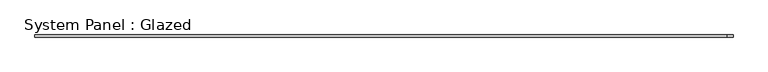
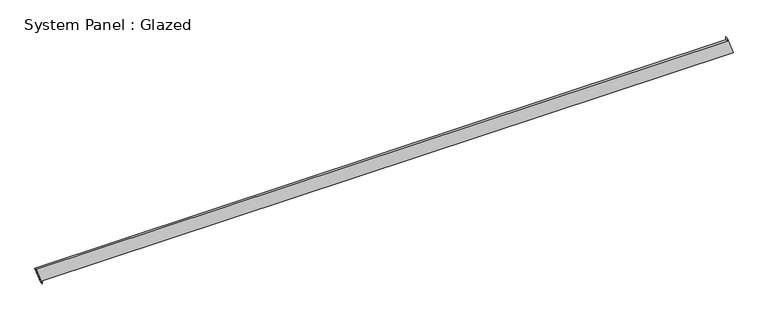
"""IFC4 building model written with IfcOpenShell, lengths in millimetres: plate geometry, System Panel : Glazed."""

from ifc_helpers import new_model, si_unit, frame, origin, place, context, project, spatial, polyline, outline, extrude, source, transform, mapped, element, save


def system_panel_glazed_ea61075c(model_context):
    return source(origin(), model_context, "Body", "SweptSolid", [
        extrude(outline(polyline([(0.0, -3958.7388288), (35.3553391, -3958.7388288), (35.3553391, 4028.1708947), (235.3914127, 3958.6179308), (200.0360737, 3958.6177077), (200.0864778, -4028.1708947), (0.0, -3958.7388288)])), frame((0.0, -49.5, 0.0), z_axis=(0.0, 1.0, 0.0), x_axis=(0.0, 0.0, 1.0)), (0.0, 0.0, 1.0), 25.0),
    ])


if __name__ == "__main__":
    model = new_model("IFC4")
    model_context = context("Model", 3, world=origin())
    ifc_project = project(units=[si_unit("LENGTHUNIT", "METRE", prefix="MILLI")], contexts=[model_context])
    site = spatial("IfcSite", under=ifc_project)
    building = spatial("IfcBuilding", under=site)
    placement = place(None, origin())
    system_panel_glazed_shape = system_panel_glazed_ea61075c(model_context)
    element("IfcPlate", 1, ObjectType="System Panel : Glazed", at=placement, inside=building, context=model_context, shape_type="MappedRepresentation", body=[
        mapped(system_panel_glazed_shape, transform((0.0, 0.0, 0.0), x_axis=(1.0, 0.0, 0.0), y_axis=(0.0, 1.0, 0.0), z_axis=(0.0, 0.0, 1.0))),
    ])
    save(model, "model.ifc")

# Revit data of these elements
# Element 1 (IfcPlate, "System Panel : Glazed")
#   Materials on its faces: "Glass"
# Materials
#   "Glass": class "Glass", colour RGB 218 227 224, transparency 0.85, Description = "Soda Lime Glass", Cost = 0
